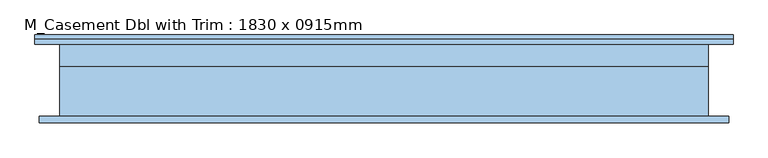
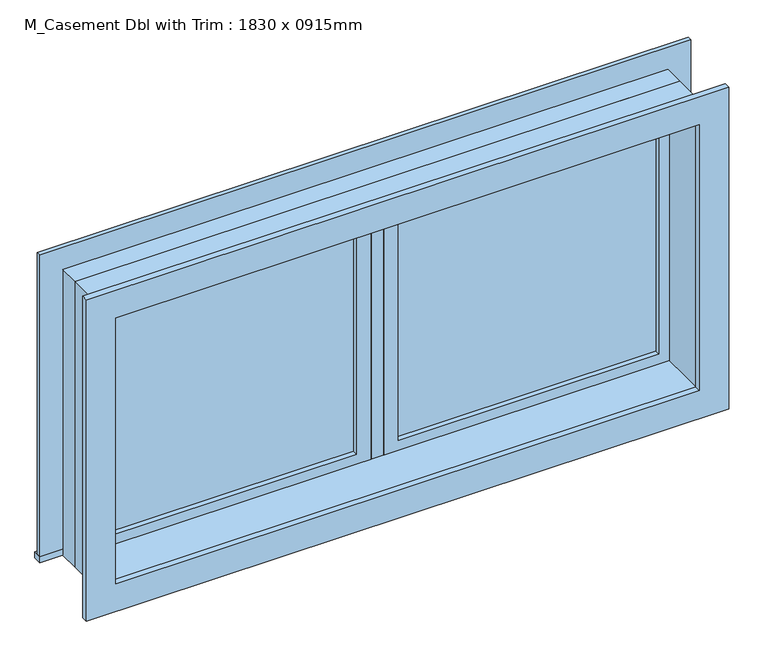
"""IFC4 building model written with IfcOpenShell, lengths in millimetres: window geometry, M_Casement Dbl with Trim : 1830 x 0915mm."""

from ifc_helpers import new_model, si_unit, frame, origin, place, context, project, spatial, polyline, outline, extrude, source, transform, mapped, element, save


def m_casement_dbl_with_trim_1830_x_0915mm_5bb5ad82(model_context):
    return source(origin(), model_context, "Body", "SweptSolid", [
        extrude(outline(polyline([(63.5, 85.775), (851.5, 85.775), (851.5, 73.075), (63.5, 73.075), (63.5, 85.775)])), frame((0.0, 0.0, 1283.5), z_axis=(0.0, 0.0, 1.0), x_axis=(1.0, 0.0, 0.0)), (0.0, 0.0, 1.0), 788.0),
        extrude(outline(polyline([(2115.95, 19.05), (1239.05, 19.05), (1239.05, 895.95), (2115.95, 895.95), (2115.95, 19.05)]), holes=[polyline([(2071.5, 63.5), (2071.5, 851.5), (1283.5, 851.5), (1283.5, 63.5), (2071.5, 63.5)])]), frame((0.0, 57.2, 0.0), z_axis=(0.0, 1.0, 0.0), x_axis=(0.0, 0.0, 1.0)), (0.0, 0.0, 1.0), 44.45),
        extrude(outline(polyline([(-984.95, 146.35), (984.95, 146.35), (984.95, 120.65), (-984.95, 120.65), (-984.95, 146.35)])), frame((0.0, 0.0, 1220.0), z_axis=(0.0, 0.0, 1.0), x_axis=(1.0, 0.0, 0.0)), (0.0, 0.0, 1.0), 19.05),
        extrude(outline(polyline([(2115.95, -895.95), (2115.95, 895.95), (1239.05, 895.95), (1239.05, 984.95), (2204.95, 984.95), (2204.95, -984.95), (1239.05, -984.95), (1239.05, -895.95), (2115.95, -895.95)])), frame((0.0, 120.65, 0.0), z_axis=(0.0, 1.0, 0.0), x_axis=(0.0, 0.0, 1.0)), (0.0, 0.0, 1.0), 13.0),
        extrude(outline(polyline([(2192.25, 972.25), (2192.25, -972.25), (1162.75, -972.25), (1162.75, 972.25), (2192.25, 972.25)]), holes=[polyline([(2103.25, 883.25), (1251.75, 883.25), (1251.75, -883.25), (2103.25, -883.25), (2103.25, 883.25)])]), frame((0.0, -101.55, 0.0), z_axis=(0.0, 1.0, 0.0), x_axis=(0.0, 0.0, 1.0)), (0.0, 0.0, 1.0), 19.0),
        extrude(outline(polyline([(-63.5, 73.075), (-851.5, 73.075), (-851.5, 85.775), (-63.5, 85.775), (-63.5, 73.075)])), frame((0.0, 0.0, 1283.5), z_axis=(0.0, 0.0, 1.0), x_axis=(1.0, 0.0, 0.0)), (0.0, 0.0, 1.0), 788.0),
        extrude(outline(polyline([(2115.95, -895.95), (1239.05, -895.95), (1239.05, -19.05), (2115.95, -19.05), (2115.95, -895.95)]), holes=[polyline([(2071.5, -851.5), (2071.5, -63.5), (1283.5, -63.5), (1283.5, -851.5), (2071.5, -851.5)])]), frame((0.0, 57.2, 0.0), z_axis=(0.0, 1.0, 0.0), x_axis=(0.0, 0.0, 1.0)), (0.0, 0.0, 1.0), 44.45),
        extrude(outline(polyline([(2135.0, -915.0), (1220.0, -915.0), (1220.0, 915.0), (2135.0, 915.0), (2135.0, -915.0)]), holes=[polyline([(2103.25, -883.25), (2103.25, 883.25), (1251.75, 883.25), (1251.75, -883.25), (2103.25, -883.25)])]), frame((0.0, -82.55, 0.0), z_axis=(0.0, 1.0, 0.0), x_axis=(0.0, 0.0, 1.0)), (0.0, 0.0, 1.0), 139.75),
        extrude(outline(polyline([(2135.0, 915.0), (2135.0, -915.0), (1220.0, -915.0), (1220.0, 915.0), (2135.0, 915.0)]), holes=[polyline([(2115.95, 895.95), (1239.05, 895.95), (1239.05, -895.95), (2115.95, -895.95), (2115.95, 895.95)])]), frame((0.0, 57.2, 0.0), z_axis=(0.0, 1.0, 0.0), x_axis=(0.0, 0.0, 1.0)), (0.0, 0.0, 1.0), 63.45),
        extrude(outline(polyline([(19.05, 57.2), (-19.05, 57.2), (-19.05, 120.7), (19.05, 120.7), (19.05, 57.2)])), frame((0.0, 0.0, 1239.05), z_axis=(0.0, 0.0, 1.0), x_axis=(1.0, 0.0, 0.0)), (0.0, 0.0, 1.0), 876.9),
    ])


if __name__ == "__main__":
    model = new_model("IFC4")
    model_context = context("Model", 3, world=origin())
    ifc_project = project(units=[si_unit("LENGTHUNIT", "METRE", prefix="MILLI")], contexts=[model_context])
    site = spatial("IfcSite", under=ifc_project)
    building = spatial("IfcBuilding", under=site)
    placement = place(None, origin())
    m_casement_dbl_with_trim_1830_x_0915mm_shape = m_casement_dbl_with_trim_1830_x_0915mm_5bb5ad82(model_context)
    element("IfcWindow", 1, ObjectType="M_Casement Dbl with Trim : 1830 x 0915mm", at=placement, inside=building, context=model_context, shape_type="MappedRepresentation", body=[
        mapped(m_casement_dbl_with_trim_1830_x_0915mm_shape, transform((0.0, 0.0, 0.0), x_axis=(1.0, 0.0, 0.0), y_axis=(0.0, 1.0, 0.0), z_axis=(0.0, 0.0, 1.0))),
    ])
    save(model, "model.ifc")

# Revit data of these elements
# Type "M_Casement Dbl with Trim : 1830 x 0915mm"
#   Type Mark = "22"
#   Construction Type Id = "GSP4R"
#   Analytic Construction = "1/8 in Pilkington single glazing"
#   Visual Light Transmittance = 0.9
#   Solar Heat Gain Coefficient = 0.78
#   Heat Transfer Coefficient (U) = 3.6886 W/(m²·K)
#   Height = 3' - 0.02362"
#   Default Sill Height = 4' - 0.0315"
#   Trim Projection - Ext. = 0' - 0.51181"
#   Trim Projection - Int. = 0' - 0.74803"
#   Trim Width - Exterior = 0' - 3.50394"
#   Trim Width - Interior = 0' - 3.50394"
#   Width = 6' - 0.04724"
#   Window Inset = 0' - 0.74803"
#   Glass Pane Material = Glass
#   Sash = Sash
#   Trim Exterior Material = Trim
#   Trim Interior Material = Trim
#   Wall Closure = (empty or 0)
# Element 1 (IfcWindow, "M_Casement Dbl with Trim : 1830 x 0915mm")
#   Materials on its faces: "Trim", "Sash", "Glass"
# Materials
#   "Glass": class "Glass", colour RGB 0 128 192, transparency 0.75, Description = "Soda Lime Glass", Cost = 0
#   "Sash": class "Wood", colour RGB 224 178 126, transparency 0, Cost = 0
#   "Trim": class "Wood", colour RGB 224 178 126, transparency 0
